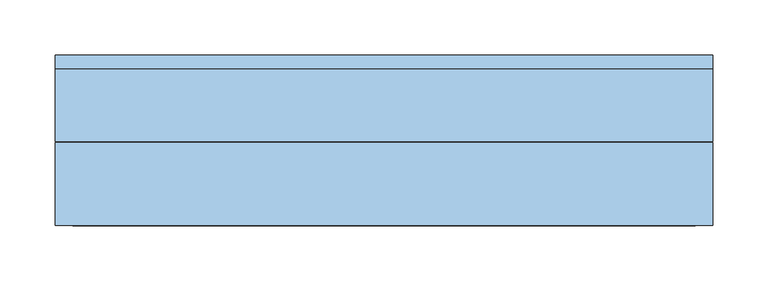
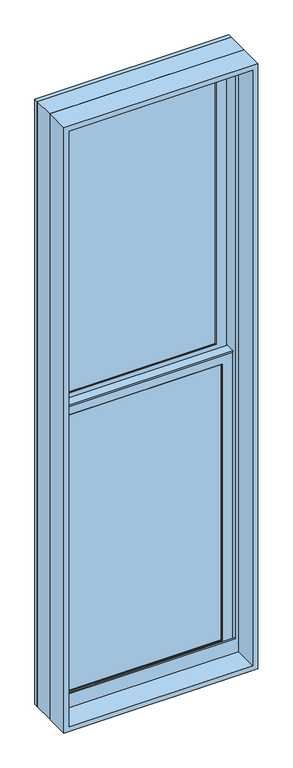
"""IFC4 building model written with IfcOpenShell, lengths in millimetres: window geometry, Window-Double_Hung-Marvin-Essential : ESDH2066."""

from ifc_helpers import new_model, si_unit, frame, origin, place, context, project, spatial, polyline, outline, extrude, faceted_brep, source, transform, mapped, element, save


def window_a4e8a833(model_context):
    return source(origin(), model_context, "Body", "SolidModel", [
        extrude(outline(polyline([(89.9583333, 20.6375), (89.9583333, 15.875), (70.9083333, 15.875), (70.9083333, 20.6375), (89.9583333, 20.6375)])), frame((0.0, 0.0, 527.05), z_axis=(0.0, 0.0, 1.0), x_axis=(1.0, 0.0, 0.0)), (0.0, 0.0, 1.0), 908.05),
        extrude(outline(polyline([(-70.9083333, 20.6375), (-70.9083333, 15.875), (-89.9583333, 15.875), (-89.9583333, 20.6375), (-70.9083333, 20.6375)])), frame((0.0, 0.0, 527.05), z_axis=(0.0, 0.0, 1.0), x_axis=(1.0, 0.0, 0.0)), (0.0, 0.0, 1.0), 908.05),
        extrude(outline(polyline([(241.3, 20.6375), (241.3, 15.875), (-241.3, 15.875), (-241.3, 20.6375), (241.3, 20.6375)])), frame((0.0, 0.0, 971.55), z_axis=(0.0, 0.0, 1.0), x_axis=(1.0, 0.0, 0.0)), (0.0, 0.0, 1.0), 19.05),
        extrude(outline(polyline([(-89.9583333, 46.83125), (-89.9583333, 51.59375), (-70.9083333, 51.59375), (-70.9083333, 46.83125), (-89.9583333, 46.83125)])), frame((0.0, 0.0, 1473.2), z_axis=(0.0, 0.0, 1.0), x_axis=(1.0, 0.0, 0.0)), (0.0, 0.0, 1.0), 908.05),
        extrude(outline(polyline([(70.9083333, 46.83125), (70.9083333, 51.59375), (89.9583333, 51.59375), (89.9583333, 46.83125), (70.9083333, 46.83125)])), frame((0.0, 0.0, 1473.2), z_axis=(0.0, 0.0, 1.0), x_axis=(1.0, 0.0, 0.0)), (0.0, 0.0, 1.0), 908.05),
        extrude(outline(polyline([(-241.3, 46.83125), (-241.3, 51.59375), (241.3, 51.59375), (241.3, 46.83125), (-241.3, 46.83125)])), frame((0.0, 0.0, 1917.7), z_axis=(0.0, 0.0, 1.0), x_axis=(1.0, 0.0, 0.0)), (0.0, 0.0, 1.0), 19.05),
        extrude(outline(polyline([(89.9583333, 20.6375), (70.9083333, 20.6375), (70.9083333, 25.4), (89.9583333, 25.4), (89.9583333, 20.6375)])), frame((0.0, 0.0, 527.05), z_axis=(0.0, 0.0, 1.0), x_axis=(1.0, 0.0, 0.0)), (0.0, 0.0, 1.0), 908.05),
        extrude(outline(polyline([(-70.9083333, 20.6375), (-89.9583333, 20.6375), (-89.9583333, 25.4), (-70.9083333, 25.4), (-70.9083333, 20.6375)])), frame((0.0, 0.0, 527.05), z_axis=(0.0, 0.0, 1.0), x_axis=(1.0, 0.0, 0.0)), (0.0, 0.0, 1.0), 908.05),
        extrude(outline(polyline([(241.3, 20.6375), (-241.3, 20.6375), (-241.3, 25.4), (241.3, 25.4), (241.3, 20.6375)])), frame((0.0, 0.0, 971.55), z_axis=(0.0, 0.0, 1.0), x_axis=(1.0, 0.0, 0.0)), (0.0, 0.0, 1.0), 19.05),
        extrude(outline(polyline([(-89.9583333, 56.35625), (-70.9083333, 56.35625), (-70.9083333, 51.59375), (-89.9583333, 51.59375), (-89.9583333, 56.35625)])), frame((0.0, 0.0, 1473.2), z_axis=(0.0, 0.0, 1.0), x_axis=(1.0, 0.0, 0.0)), (0.0, 0.0, 1.0), 908.05),
        extrude(outline(polyline([(70.9083333, 56.35625), (89.9583333, 56.35625), (89.9583333, 51.59375), (70.9083333, 51.59375), (70.9083333, 56.35625)])), frame((0.0, 0.0, 1473.2), z_axis=(0.0, 0.0, 1.0), x_axis=(1.0, 0.0, 0.0)), (0.0, 0.0, 1.0), 908.05),
        extrude(outline(polyline([(-241.3, 56.35625), (241.3, 56.35625), (241.3, 51.59375), (-241.3, 51.59375), (-241.3, 56.35625)])), frame((0.0, 0.0, 1917.7), z_axis=(0.0, 0.0, 1.0), x_axis=(1.0, 0.0, 0.0)), (0.0, 0.0, 1.0), 19.05),
        faceted_brep([(-268.2875, 5.6780605, 1465.1351748), (-268.2875, 5.6780605, 1460.5), (268.2875, 5.6780605, 1460.5), (268.2875, 5.6780605, 1465.1351748), (-268.2875, 34.8118605, 1465.1351748), (268.2875, 34.8118605, 1465.1351748), (268.2875, 34.8118605, 1460.5), (-268.2875, 34.8118605, 1460.5), (-268.2875, 30.1625, 1460.5), (-268.2875, 30.1625, 500.0625), (-268.2875, 8.9241104, 500.0625), (-268.2875, 8.9241104, 1460.5), (268.2875, 8.9241104, 1460.5), (268.2875, 30.1625, 1460.5), (268.2875, 8.9241104, 500.0625), (268.2875, 30.1625, 500.0625), (-252.4034752, 11.90625, 1446.2034752), (-252.4034752, 30.1625, 1446.2034752), (252.4034752, 30.1625, 1446.2034752), (252.4034752, 11.90625, 1446.2034752), (-235.74375, 10.4662439, 1429.54375), (-235.74375, 11.90625, 1429.54375), (235.74375, 11.90625, 1429.54375), (235.74375, 10.4662439, 1429.54375), (237.2858834, 8.9241104, 1431.0858834), (-237.2858834, 8.9241104, 1431.0858834), (252.4034752, 30.1625, 515.9465248), (252.4034752, 11.90625, 515.9465248), (235.74375, 11.90625, 532.60625), (235.74375, 10.4662439, 532.60625), (237.2858834, 8.9241104, 531.0641166), (-252.4034752, 30.1625, 515.9465248), (-252.4034752, 11.90625, 515.9465248), (-235.74375, 11.90625, 532.60625), (-235.74375, 10.4662439, 532.60625), (-237.2858834, 8.9241104, 531.0641166)], [[[0, 1, 2, 3]], [[4, 5, 6, 7]], [[1, 0, 4, 7, 8, 9, 10, 11]], [[2, 1, 11, 12]], [[7, 6, 13, 8]], [[3, 2, 12, 14, 15, 13, 6, 5]], [[0, 3, 5, 4]], [[16, 17, 18, 19]], [[20, 21, 22, 23]], [[20, 23, 24, 25]], [[19, 18, 26, 27]], [[23, 22, 28, 29]], [[24, 23, 29, 30]], [[27, 26, 31, 32]], [[29, 28, 33, 34]], [[30, 29, 34, 35]], [[15, 14, 10, 9]], [[15, 9, 8, 13], [18, 17, 31, 26]], [[17, 16, 32, 31]], [[16, 19, 27, 32], [22, 21, 33, 28]], [[21, 20, 34, 33]], [[20, 25, 35, 34]], [[10, 14, 12, 11], [25, 24, 30, 35]]]),
        extrude(outline(polyline([(38.5955581, 1446.2125), (33.5778968, 1446.2125), (33.5778968, 1447.8), (39.9405976, 1447.8), (39.9405976, 1446.2125), (61.515625, 1446.2125), (47.6307501, 1442.8975159), (38.5955581, 1442.8975159), (38.5955581, 1446.2125)])), frame((-268.2875, 0.0, 0.0), z_axis=(1.0, 0.0, 0.0), x_axis=(0.0, 1.0, 0.0)), (0.0, 0.0, 1.0), 536.575),
        faceted_brep([(298.45, 0.0, 469.9), (298.45, 0.0, 2438.4), (-298.45, 0.0, 2438.4), (-298.45, 0.0, 469.9), (272.25625, 0.0, 531.01875), (-272.25625, 0.0, 531.01875), (-272.25625, 0.0, 2412.20625), (272.25625, 0.0, 2412.20625), (272.25625, 3.96875, 469.9), (-272.25625, 3.96875, 469.9), (-272.25625, 3.96875, 531.01875), (272.25625, 3.96875, 531.01875), (-298.45, 65.6828125, 469.9), (-272.25625, 65.6828125, 469.9), (272.25625, 65.6828125, 469.9), (298.45, 65.6828125, 469.9), (-298.45, 65.6828125, 2438.4), (298.45, 65.6828125, 2438.4), (272.25625, 65.6828125, 2412.20625), (-272.25625, 65.6828125, 2412.20625)], [[[0, 1, 2, 3], [4, 5, 6, 7]], [[8, 9, 10, 11]], [[5, 4, 11, 10]], [[0, 3, 12, 13, 9, 8, 14, 15]], [[13, 12, 16, 17, 15, 14, 18, 19]], [[13, 19, 6, 5, 10, 9]], [[7, 6, 19, 18]], [[18, 14, 8, 11, 4, 7]], [[1, 0, 15, 17]], [[2, 1, 17, 16]], [[3, 2, 16, 12]]]),
        faceted_brep([(272.25625, 30.1625, 1454.15), (270.66875, 30.1625, 1454.15), (270.66875, 30.1625, 494.2544613), (272.25625, 30.1625, 494.2544613), (-270.66875, 30.1625, 1454.15), (-272.25625, 30.1625, 1454.15), (-272.25625, 30.1625, 494.2544613), (-270.66875, 30.1625, 494.2544613), (270.66875, 63.5, 1454.15), (272.25625, 63.5, 1454.15), (272.25625, 63.5, 487.7743077), (270.66875, 63.5, 487.7743077), (-272.25625, 63.5, 1454.15), (-270.66875, 63.5, 1454.15), (-270.66875, 63.5, 487.7743077), (-272.25625, 63.5, 487.7743077), (283.5108932, 3.96875, 499.3460105), (283.5108932, 3.96875, 469.9), (283.5108932, 65.6828125, 469.9), (283.5108932, 65.6828125, 487.350012), (-283.5108932, 3.96875, 469.9), (-283.5108932, 3.96875, 499.3460105), (-283.5108932, 65.6828125, 487.350012), (-283.5108932, 65.6828125, 469.9), (283.5108932, 78.58125, 484.8428097), (-283.5108932, 78.58125, 484.8428097), (-281.4971252, 68.2348864, 486.8539391), (-263.53135, 68.2348864, 486.8539391), (-263.53135, 65.6828125, 487.350012), (263.53135, 65.6828125, 487.350012), (263.53135, 68.2348864, 486.8539391), (281.4971252, 68.2348864, 486.8539391), (-298.45, 65.6828125, 469.9), (-298.45, 78.5948249, 469.9), (298.45, 78.5948249, 469.9), (298.45, 65.6828125, 469.9), (-298.45, 78.58125, 2438.4), (298.45, 78.58125, 2438.4), (283.5108932, 78.58125, 2423.4608932), (-283.5108932, 78.58125, 2423.4608932), (-298.45, 65.6828125, 2438.4), (-281.4971252, 68.2348864, 2421.4471252), (281.4971252, 68.2348864, 2421.4471252), (263.53135, 68.2348864, 2403.48135), (-263.53135, 68.2348864, 2403.48135), (-263.53135, 65.6828125, 2403.48135), (263.53135, 65.6828125, 2403.48135), (298.45, 65.6828125, 2438.4)], [[[0, 1, 2, 3]], [[4, 5, 6, 7]], [[8, 9, 10, 11]], [[12, 13, 14, 15]], [[1, 8, 11, 2]], [[9, 0, 3, 10]], [[1, 0, 9, 8]], [[5, 4, 13, 12]], [[5, 12, 15, 6]], [[13, 4, 7, 14]], [[16, 17, 18, 19]], [[20, 21, 22, 23]], [[24, 25, 26, 27, 28, 22, 21, 16, 19, 29, 30, 31], [3, 2, 11, 10], [7, 6, 15, 14]], [[17, 16, 21, 20]], [[17, 20, 23, 32, 33, 34, 35, 18]], [[34, 33, 36, 37], [25, 24, 38, 39]], [[33, 32, 40, 36]], [[39, 41, 26, 25]], [[41, 42, 31, 30, 43, 44, 27, 26]], [[44, 45, 28, 27]], [[40, 32, 23, 22, 28, 45, 46, 29, 19, 18, 35, 47]], [[36, 40, 47, 37]], [[39, 38, 42, 41]], [[44, 43, 46, 45]], [[34, 37, 47, 35]], [[42, 38, 24, 31]], [[46, 43, 30, 29]]]),
        extrude(outline(polyline([(248.44375, 11.90625), (-248.44375, 11.90625), (-248.44375, 15.08125), (248.44375, 15.08125), (248.44375, 11.90625)])), frame((0.0, 0.0, 519.90625), z_axis=(0.0, 0.0, 1.0), x_axis=(1.0, 0.0, 0.0)), (0.0, 0.0, 1.0), 922.3375),
        extrude(outline(polyline([(248.44375, 42.8625), (-248.44375, 42.8625), (-248.44375, 46.0375), (248.44375, 46.0375), (248.44375, 42.8625)])), frame((0.0, 0.0, 1466.05625), z_axis=(0.0, 0.0, 1.0), x_axis=(1.0, 0.0, 0.0)), (0.0, 0.0, 1.0), 922.3375),
        faceted_brep([(-235.74375, 31.194477, 1429.54375), (-237.2858834, 32.7366104, 1431.0858834), (237.2858834, 32.7366104, 1431.0858834), (235.74375, 31.194477, 1429.54375), (-235.74375, 30.1625, 1429.54375), (235.74375, 30.1625, 1429.54375), (-268.2875, 32.7366104, 1462.0875), (-268.2875, 30.1625, 1462.0875), (268.2875, 30.1625, 1462.0875), (268.2875, 32.7366104, 1462.0875), (237.2858834, 32.7366104, 531.0641166), (235.74375, 31.194477, 532.60625), (235.74375, 30.1625, 532.60625), (268.2875, 30.1625, 500.0625), (268.2875, 32.7366104, 500.0625), (-237.2858834, 32.7366104, 531.0641166), (-235.74375, 31.194477, 532.60625), (-235.74375, 30.1625, 532.60625), (-268.2875, 30.1625, 500.0625), (-268.2875, 32.7366104, 500.0625)], [[[0, 1, 2, 3]], [[4, 0, 3, 5]], [[6, 7, 8, 9]], [[3, 2, 10, 11]], [[5, 3, 11, 12]], [[9, 8, 13, 14]], [[11, 10, 15, 16]], [[12, 11, 16, 17]], [[14, 13, 18, 19]], [[9, 14, 19, 6], [1, 15, 10, 2]], [[16, 15, 1, 0]], [[17, 16, 0, 4]], [[7, 18, 13, 8], [5, 12, 17, 4]], [[19, 18, 7, 6]]]),
        faceted_brep([(-252.4034752, 42.8625, 2392.3534752), (-252.4034752, 61.11875, 2392.3534752), (252.4034752, 61.11875, 2392.3534752), (252.4034752, 42.8625, 2392.3534752), (-235.74375, 41.4224939, 2375.69375), (-235.74375, 42.8625, 2375.69375), (235.74375, 42.8625, 2375.69375), (235.74375, 41.4224939, 2375.69375), (-237.2858834, 39.8803604, 2377.2358834), (237.2858834, 39.8803604, 2377.2358834), (-268.2875, 61.11875, 2408.2375), (-268.2875, 39.8803604, 2408.2375), (268.2875, 39.8803604, 2408.2375), (268.2875, 61.11875, 2408.2375), (252.4034752, 61.11875, 1462.0965248), (252.4034752, 42.8625, 1462.0965248), (235.74375, 42.8625, 1478.75625), (235.74375, 41.4224939, 1478.75625), (237.2858834, 39.8803604, 1477.2141166), (268.2875, 39.8803604, 1446.2125), (268.2875, 61.11875, 1446.2125), (-252.4034752, 61.11875, 1462.0965248), (-252.4034752, 42.8625, 1462.0965248), (-235.74375, 42.8625, 1478.75625), (-235.74375, 41.4224939, 1478.75625), (-237.2858834, 39.8803604, 1477.2141166), (-268.2875, 39.8803604, 1446.2125), (-268.2875, 61.11875, 1446.2125)], [[[0, 1, 2, 3]], [[4, 5, 6, 7]], [[8, 4, 7, 9]], [[10, 11, 12, 13]], [[3, 2, 14, 15]], [[7, 6, 16, 17]], [[9, 7, 17, 18]], [[13, 12, 19, 20]], [[15, 14, 21, 22]], [[17, 16, 23, 24]], [[18, 17, 24, 25]], [[20, 19, 26, 27]], [[13, 20, 27, 10], [1, 21, 14, 2]], [[22, 21, 1, 0]], [[3, 15, 22, 0], [5, 23, 16, 6]], [[24, 23, 5, 4]], [[25, 24, 4, 8]], [[11, 26, 19, 12], [9, 18, 25, 8]], [[27, 26, 11, 10]]]),
        faceted_brep([(-268.2875, 61.11875, 1446.2125), (-268.2875, 63.6928604, 1446.2125), (268.2875, 63.6928604, 1446.2125), (268.2875, 61.11875, 1446.2125), (-235.74375, 62.150727, 1478.75625), (-235.74375, 61.11875, 1478.75625), (235.74375, 61.11875, 1478.75625), (235.74375, 62.150727, 1478.75625), (-237.2858834, 63.6928604, 1477.2141166), (237.2858834, 63.6928604, 1477.2141166), (268.2875, 63.6928604, 2408.2375), (268.2875, 61.11875, 2408.2375), (235.74375, 61.11875, 2375.69375), (235.74375, 62.150727, 2375.69375), (237.2858834, 63.6928604, 2377.2358834), (-268.2875, 63.6928604, 2408.2375), (-268.2875, 61.11875, 2408.2375), (-235.74375, 61.11875, 2375.69375), (-235.74375, 62.150727, 2375.69375), (-237.2858834, 63.6928604, 2377.2358834)], [[[0, 1, 2, 3]], [[4, 5, 6, 7]], [[8, 4, 7, 9]], [[3, 2, 10, 11]], [[7, 6, 12, 13]], [[9, 7, 13, 14]], [[11, 10, 15, 16]], [[13, 12, 17, 18]], [[14, 13, 18, 19]], [[16, 15, 1, 0]], [[3, 11, 16, 0], [5, 17, 12, 6]], [[18, 17, 5, 4]], [[19, 18, 4, 8]], [[1, 15, 10, 2], [9, 14, 19, 8]]]),
        extrude(outline(polyline([(248.44375, 26.19375), (-248.44375, 26.19375), (-248.44375, 30.1625), (248.44375, 30.1625), (248.44375, 26.19375)])), frame((0.0, 0.0, 519.90625), z_axis=(0.0, 0.0, 1.0), x_axis=(1.0, 0.0, 0.0)), (0.0, 0.0, 1.0), 922.3375),
        extrude(outline(polyline([(248.44375, 57.15), (-248.44375, 57.15), (-248.44375, 61.11875), (248.44375, 61.11875), (248.44375, 57.15)])), frame((0.0, 0.0, 1466.05625), z_axis=(0.0, 0.0, 1.0), x_axis=(1.0, 0.0, 0.0)), (0.0, 0.0, 1.0), 922.3375),
        extrude(outline(polyline([(2438.4, 298.45), (2438.4, -298.45), (469.9, -298.45), (469.9, 298.45), (2438.4, 298.45)]), holes=[polyline([(2422.525, 282.575), (485.775, 282.575), (485.775, -282.575), (2422.525, -282.575), (2422.525, 282.575)])]), frame((0.0, -76.2, 0.0), z_axis=(0.0, 1.0, 0.0), x_axis=(0.0, 0.0, 1.0)), (0.0, 0.0, 1.0), 75.40625),
    ])


if __name__ == "__main__":
    model = new_model("IFC4")
    model_context = context("Model", 3, world=origin())
    ifc_project = project(units=[si_unit("LENGTHUNIT", "METRE", prefix="MILLI")], contexts=[model_context])
    site = spatial("IfcSite", under=ifc_project)
    building = spatial("IfcBuilding", under=site)
    placement = place(None, origin())
    window_shape = window_a4e8a833(model_context)
    element("IfcWindow", 1, ObjectType="Window-Double_Hung-Marvin-Essential : ESDH2066", at=placement, inside=building, context=model_context, shape_type="MappedRepresentation", body=[
        mapped(window_shape, transform((0.0, 0.0, 0.0), x_axis=(1.0, 0.0, 0.0), y_axis=(0.0, 1.0, 0.0), z_axis=(0.0, 0.0, 1.0))),
    ])
    save(model, "model.ifc")

# Revit data of these elements
# Type "Window-Double_Hung-Marvin-Essential : ESDH2066"
#   Type Mark = "83"
#   Window Type = "Essential Double Hung"
#   Product data url = "https://bimobject.com/marvin-windows-and-doors/product/marvin-dhwau"
#   Product Guid = "c4a96547-874c-4385-91dc-a058adc19d98"
#   Frame = "All Ultrex"
#   Egress Window = "No"
#   URL = "www.marvin.com"
#   Model = "ESDH2066"
#   Manufacturer = "Marvin Windows and Doors"
#   Label Egress = ""
#   Glass Type = "IG Low E II with Argon"
#   Design Pressure = "DP40"
#   Description = "2478 DBHG"
#   Analytic Construction = "<None>"
#   Prairie Corner Width = 0' - 4"
#   Prairie Corner Height = 0' - 4"
#   Egress Width = 1' - 8 9/16"
#   Egress Height = 2' - 10 27/128"
#   Rough Width = 2' - 0"
#   Rough Height = 6' - 6"
#   Nominal Width = 2' - 0"
#   Nominal Height = 6' - 6"
#   Inset to Installation Flange [instance default] = 0' - 1"
#   Height = 6' - 5 1/2"
#   Egress Area = 4.88516 SF
#   Default Head Height = 8' - 0"
#   Width = 1' - 11 1/2"
#   Daylight Area = 9.104 SF
#   DLO Width = 1' - 6 9/16"
#   DLO Height = 2' - 11 5/16"
#   Muntins Top Sash = yes
#   Lites Wide Top Sash = 3
#   Lites Wide Bottom Sash = 3
#   Lites High Top Sash = 2
#   Lites High Bottom Sash = 2
#   Lite Cut Prairie 9 = no
#   Lite Cut HV Grid = yes
#   Muntins Bottom Sash = yes
#   Label Visibility = no
#   Jamb Extension Visibility = yes
#   Edition number = 1
#   Interior Material = Ultrex-Marvin-Stonewhite
#   Glazing Material = Glass-Marvin-IG Low E II with Argon
#   Cladding Material = Ultrex-Marvin-Pebblegray
#   Wall Closure = (empty or 0)
#   Assembly Code = ""
# Element 1 (IfcWindow, "Window-Double_Hung-Marvin-Essential : ESDH2066")
#   Materials on its faces: "Ultrex-Marvin-Pebblegray", "Ultrex-Marvin-Stonewhite", "Glass-Marvin-IG Low E II with Argon"
# Materials
#   "Ultrex-Marvin-Stonewhite": class "Paint", colour RGB 250 251 245, transparency 0
#   "Glass-Marvin-IG Low E II with Argon": class "Glass", colour RGB 0 128 192, transparency 0.85
#   "Ultrex-Marvin-Pebblegray": class "Paint", colour RGB 189 185 173, transparency 0
